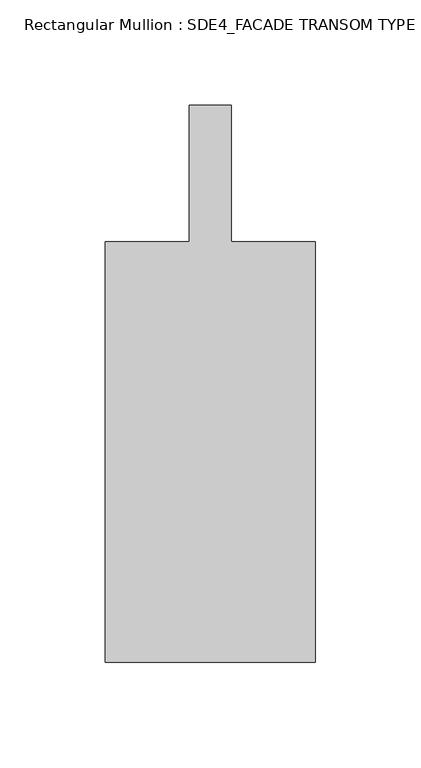
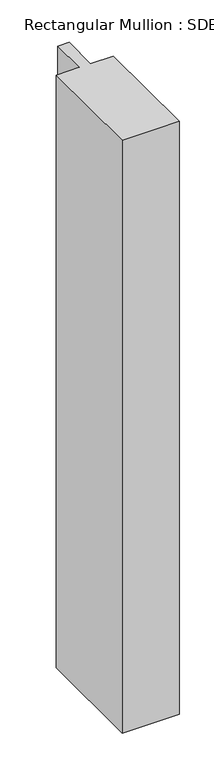
"""IFC4 building model written with IfcOpenShell, lengths in millimetres: member geometry, Rectangular Mullion : SDE4_FACADE TRANSOM TYPE 2."""

from ifc_helpers import new_model, si_unit, frame, origin, place, context, project, spatial, polyline, outline, extrude, source, transform, mapped, element, save


def rectangular_mullion_sde4_facade_transom_type_2_c090c89a(model_context):
    return source(origin(), model_context, "Body", "SweptSolid", [
        extrude(outline(polyline([(50.0, -132.5), (-50.0, -132.5), (-50.0, 67.5), (-10.0, 67.5), (-10.0, 132.5), (10.0, 132.5), (10.0, 67.5), (50.0, 67.5), (50.0, -132.5)])), frame((0.0, 0.0, -1100.0000004), z_axis=(0.0, 0.0, 1.0), x_axis=(1.0, 0.0, 0.0)), (0.0, 0.0, 1.0), 1100.0000004),
    ])


if __name__ == "__main__":
    model = new_model("IFC4")
    model_context = context("Model", 3, world=origin())
    ifc_project = project(units=[si_unit("LENGTHUNIT", "METRE", prefix="MILLI")], contexts=[model_context])
    site = spatial("IfcSite", under=ifc_project)
    building = spatial("IfcBuilding", under=site)
    placement = place(None, origin())
    rectangular_mullion_sde4_facade_transom_type_2_shape = rectangular_mullion_sde4_facade_transom_type_2_c090c89a(model_context)
    element("IfcMember", 1, ObjectType="Rectangular Mullion : SDE4_FACADE TRANSOM TYPE 2", at=placement, inside=building, context=model_context, shape_type="MappedRepresentation", body=[
        mapped(rectangular_mullion_sde4_facade_transom_type_2_shape, transform((0.0, 0.0, 0.0), x_axis=(1.0, 0.0, 0.0), y_axis=(0.0, 1.0, 0.0), z_axis=(0.0, 0.0, 1.0))),
    ])
    save(model, "model.ifc")

# Revit data of these elements
# Type "Rectangular Mullion : SDE4_FACADE TRANSOM TYPE 2"
#   built-in parameter 1007322 = 0.869423 (stored number, unit not read)
#   built-in parameter 1007321 = 0.164042 (stored number, unit not read)
#   built-in parameter 1007320 = 0.164042 (stored number, unit not read)
